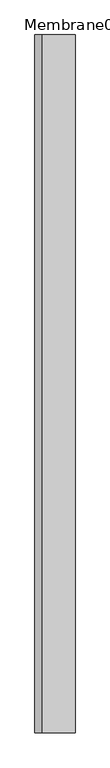
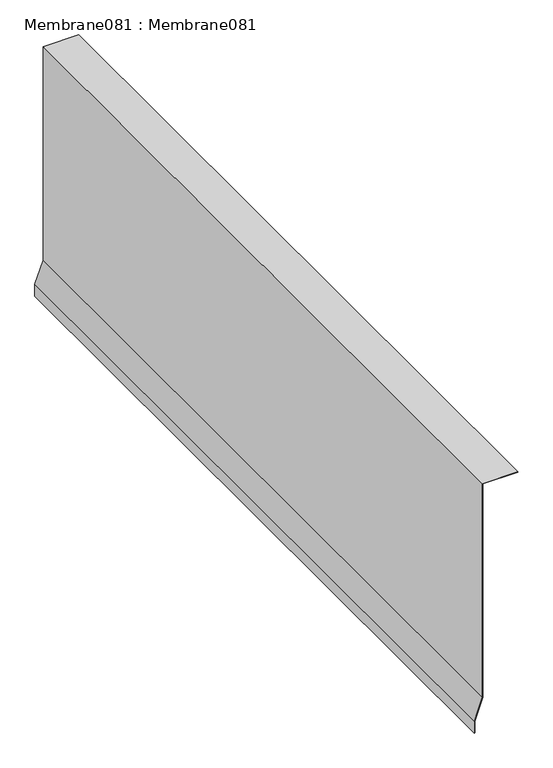
"""IFC4 building model written with IfcOpenShell, lengths in millimetres: proxy geometry, Membrane081 : Membrane081."""

from ifc_helpers import new_model, si_unit, frame, origin, place, context, project, spatial, polyline, outline, extrude, source, transform, mapped, element, save


def membrane081_membrane081_5ac18572(model_context):
    return source(origin(), model_context, "Body", "SweptSolid", [
        extrude(outline(polyline([(40237.828125, -2674.0896171), (40237.828125, -2767.6617221), (39645.0411306, -2767.6617221), (39585.9385394, -2789.1733061), (39552.6918208, -2789.1733061), (39552.6918208, -2788.1733061), (39585.7622124, -2788.1733061), (39644.8648036, -2766.6617221), (40236.828125, -2766.6617221), (40236.828125, -2674.0896171), (40237.828125, -2674.0896171)])), frame((0.0, 999.7499999, 0.0), z_axis=(0.0, 1.0, 0.0), x_axis=(0.0, 0.0, 1.0)), (0.0, 0.0, 1.0), 2000.0),
    ])


if __name__ == "__main__":
    model = new_model("IFC4")
    model_context = context("Model", 3, world=origin())
    ifc_project = project(units=[si_unit("LENGTHUNIT", "METRE", prefix="MILLI")], contexts=[model_context])
    site = spatial("IfcSite", under=ifc_project)
    building = spatial("IfcBuilding", under=site)
    placement = place(None, origin())
    membrane081_membrane081_shape = membrane081_membrane081_5ac18572(model_context)
    element("IfcBuildingElementProxy", 1, Name="Membrane081 : Membrane081", ObjectType="Membrane081 : Membrane081", at=placement, inside=building, context=model_context, shape_type="MappedRepresentation", body=[
        mapped(membrane081_membrane081_shape, transform((0.0, 0.0, 0.0), x_axis=(1.0, 0.0, 0.0), y_axis=(0.0, 1.0, 0.0), z_axis=(0.0, 0.0, 1.0))),
    ])
    save(model, "model.ifc")

# Revit data of these elements
# Type "Membrane081 : Membrane081"
#   NameOverride = "Membrane081"
# Element 1 (IfcBuildingElementProxy, "Membrane081 : Membrane081")
#   Materials on its faces: "(2) LAYERS OF ICE & WATER SHIELD (BITUTHANE) UNDER STUCCO"
# Materials
#   "(2) LAYERS OF ICE & WATER SHIELD (BITUTHANE) UNDER STUCCO": class "Unassigned", colour RGB 186 255 159, transparency 0, Cost = 0
